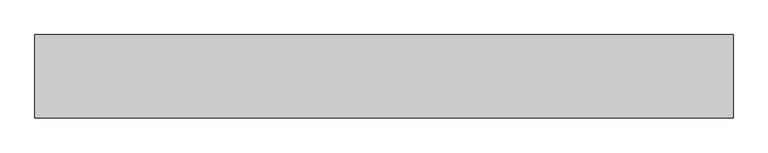
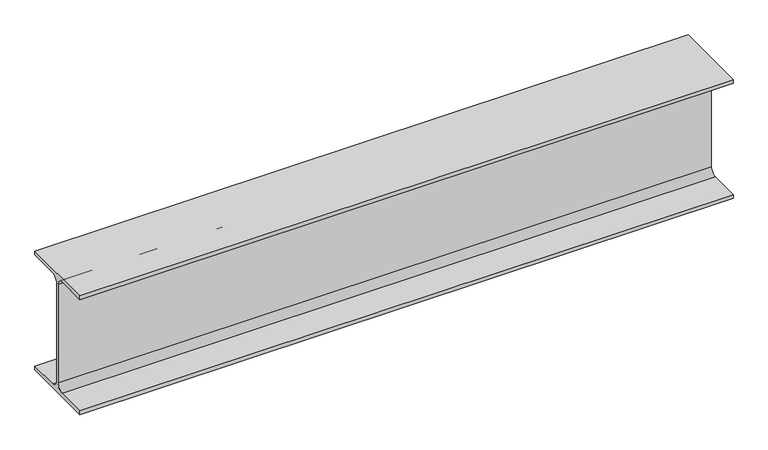
"""IFC4 building model written with IfcOpenShell, lengths in millimetres: beam geometry, 0912_Steel Framing_H-KSD3502 : H_SB_ASB_H-482x300x11x15."""

from ifc_helpers import new_model, si_unit, point, frame, frame_2d, origin, place, context, project, spatial, polyline, circle_curve, trimmed, segment, composite_curve, outline, extrude, source, transform, mapped, element, save


def beam_3e3a8e78(model_context):
    return source(origin(), model_context, "Body", "SweptSolid", [
        extrude(outline(composite_curve([segment(polyline([(150.0, -226.0), (150.0, -241.0), (-150.0, -241.0), (-150.0, -226.0), (-31.5, -226.0)]), True, "CONTINUOUS"), segment(trimmed(circle_curve(frame_2d((-31.5, -200.0)), 26.0), [point((-31.5, -226.0))], [point((-5.5, -200.0))], True, "CARTESIAN"), True, "CONTINUOUS"), segment(polyline([(-5.5, -200.0), (-5.5, 200.0)]), True, "CONTINUOUS"), segment(trimmed(circle_curve(frame_2d((-31.5, 200.0)), 26.0), [point((-5.5, 200.0))], [point((-31.5, 226.0))], True, "CARTESIAN"), True, "CONTINUOUS"), segment(polyline([(-31.5, 226.0), (-150.0, 226.0), (-150.0, 241.0), (150.0, 241.0), (150.0, 226.0), (31.5, 226.0)]), True, "CONTINUOUS"), segment(trimmed(circle_curve(frame_2d((31.5, 200.0)), 26.0), [point((31.5, 226.0))], [point((5.5, 200.0))], True, "CARTESIAN"), True, "CONTINUOUS"), segment(polyline([(5.5, 200.0), (5.5, -200.0)]), True, "CONTINUOUS"), segment(trimmed(circle_curve(frame_2d((31.5, -200.0)), 26.0), [point((5.5, -200.0))], [point((31.5, -226.0))], True, "CARTESIAN"), True, "CONTINUOUS"), segment(polyline([(31.5, -226.0), (150.0, -226.0)]), True, "CONTINUOUS")], self_intersect=False)), frame((-1254.8, 0.0, 0.0), z_axis=(1.0, 0.0, 0.0), x_axis=(0.0, 1.0, 0.0)), (0.0, 0.0, 1.0), 2509.6),
    ])


if __name__ == "__main__":
    model = new_model("IFC4")
    model_context = context("Model", 3, world=origin())
    ifc_project = project(units=[si_unit("LENGTHUNIT", "METRE", prefix="MILLI")], contexts=[model_context])
    site = spatial("IfcSite", under=ifc_project)
    building = spatial("IfcBuilding", under=site)
    placement = place(None, origin())
    beam_shape = beam_3e3a8e78(model_context)
    element("IfcBeam", 1, ObjectType="0912_Steel Framing_H-KSD3502 : H_SB_ASB_H-482x300x11x15", at=placement, inside=building, context=model_context, shape_type="MappedRepresentation", body=[
        mapped(beam_shape, transform((0.0, 0.0, 0.0), x_axis=(1.0, 0.0, 0.0), y_axis=(0.0, 1.0, 0.0), z_axis=(0.0, 0.0, 1.0))),
    ])
    save(model, "model.ifc")

# Revit data of these elements
# Type "0912_Steel Framing_H-KSD3502 : H_SB_ASB_H-482x300x11x15"
#   H_WM Code_1 = "S01AA001-00001 | Main Steel Structure Fabrication Work | Shelter/Building | Heavy Steel - Standard (Weight≥90KG/M) | Material: (   )"
#   H_WM Code_2 = "S03AA027-00001 | Main Steel Structure Erection Work | Shelter/Building | Heavy Steel (Weight≥90KG/M) | Material: (   )"
#   H_WM Code_3 = "S01AA010-00001 | Main Steel Structure Fabrication Work | Shelter/Building | Steel Painting/Coating | for Non-Fireproofed Steel Surface, Surface Preparation, Primer, Second & Final Coat | Material: (   )"
#   H_Q'ty Cal Type Tag = "SB-Q2"
#   Width = 30.0 cm
#   Web Thickness = 1.1 cm
#   Web Fillet = 2.6 cm
#   Warping Constant = 3680000.0 cm⁶
#   W = 0
#   Torsional Moment of Inertia = 88.2192 cm⁴
#   Section Area = 145.5 cm²
#   Plastic Modulus weak axis = 695.0 cm³
#   Plastic Modulus strong axis = 2790.0 cm³
#   Perimeter = 2.10 m²/m
#   Nominal Weight = 114.00 kgf/m
#   Moment of Inertia weak axis = 6760.00 cm⁴
#   Moment of Inertia strong axis = 60400.00 cm⁴
#   Height = 48.2 cm
#   Flange Thickness = 1.5 cm
#   Elastic Modulus weak axis = 451.0 cm³
#   Elastic Modulus strong axis = 2500.0 cm³
#   Centroid Vertical = 24.1 cm
#   Centroid Horizontal = 15.0 cm
#   Ix = 604000000
#   Length [instance default] = 1.5240 m
#   Zx = 2790000
#   b = 0.3000 m
#   h = 0.4820 m
#   r = 0.0260 m
#   s = 0.0110 m
#   t = 0.0150 m
#   A = 0.01455 m²
#   Structural Material [instance default] = Steel, 45-345
#   Assembly Code = ""
# Element 1 (IfcBeam, "0912_Steel Framing_H-KSD3502 : H_SB_ASB_H-482x300x11x15")
#   Structural Material = none
# Materials
#   "Steel, 45-345": class "Metal", colour RGB 189 187 185, transparency 0, Description = "Steel 345 MPa", Cost = 0
